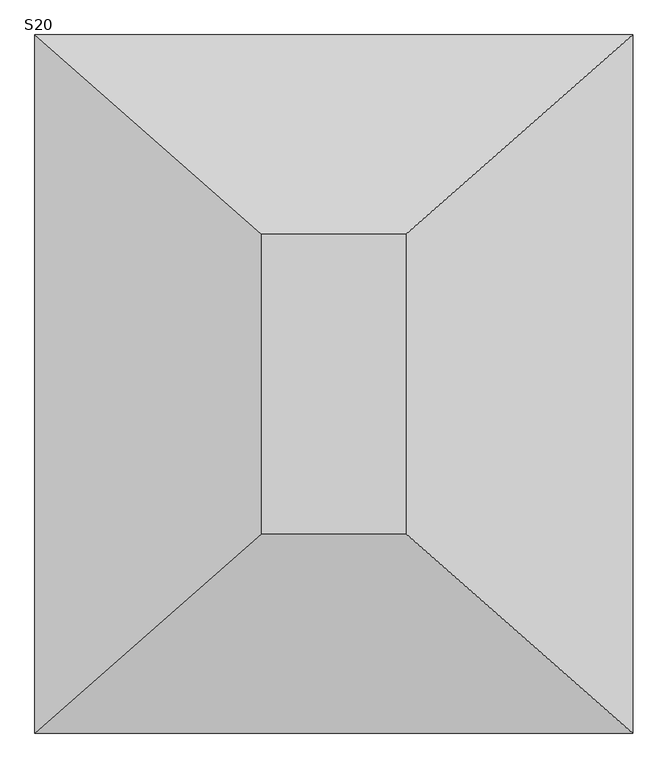
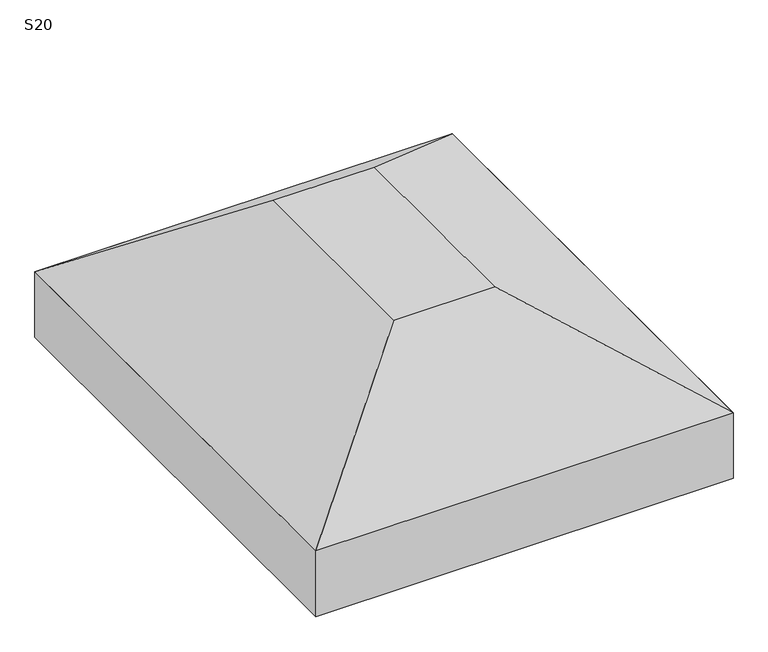
"""IFC4 building model written with IfcOpenShell, lengths in millimetres: fastener geometry, TQS - Sapata : S20."""

import ifcopenshell
import ifcopenshell.guid

model = None  # the IFC model being written
_history = None  # IfcOwnerHistory: only IFC2X3 demands one
_inside = {}  # id of a spatial element -> (the spatial element, [elements in it])
_under = {}  # id of a project, library or spatial element -> (it, [spatial elements below it])
_declared = {}  # id of a project -> (the project, [libraries it declares])
_typed = {}  # id of a type object -> (the type object, [elements of that type])
_made_of = {}  # id of a material, layer set ... -> (it, [elements and type objects made of it])


def new_model(schema):
    """Start an empty IFC model of exactly this schema.

    Asked for "IFC4X3", IfcOpenShell would pick the latest addendum, in which some entities
    have other attributes; the version numbers below select the first issue.
    IFC2X3 requires an IfcOwnerHistory on every rooted entity: one is made here for all.
    """
    global model, _history
    if schema == "IFC4X3":
        model = ifcopenshell.file(schema_version=(4, 3, 0, 0))
    else:
        model = ifcopenshell.file(schema=schema)
    _inside.clear()
    _under.clear()
    _declared.clear()
    _typed.clear()
    _made_of.clear()
    _history = None
    if model.schema == "IFC2X3":
        org = make("IfcOrganization", Name="unknown")
        user = make(
            "IfcPersonAndOrganization",
            ThePerson=make("IfcPerson", FamilyName="unknown"),
            TheOrganization=org,
        )
        app = make(
            "IfcApplication",
            ApplicationDeveloper=org,
            Version="unknown",
            ApplicationFullName="unknown",
            ApplicationIdentifier="unknown",
        )
        _history = make(
            "IfcOwnerHistory",
            OwningUser=user,
            OwningApplication=app,
            ChangeAction="ADDED",
            CreationDate=0,
        )
    return model


def make(cls, **values):
    """One entity of the class cls with the attributes given. An attribute that is None is left unset."""
    return model.create_entity(
        cls, **{name: value for name, value in values.items() if value is not None}
    )


def rooted(cls, **values):
    """An entity with a GlobalId (a new one), such as an element, a storey or a relation."""
    return make(cls, GlobalId=ifcopenshell.guid.new(), OwnerHistory=_history, **values)


def si_unit(unit_type, name, prefix=None):
    """IfcSIUnit, for example si_unit("LENGTHUNIT", "METRE", prefix="MILLI")."""
    return make("IfcSIUnit", UnitType=unit_type, Prefix=prefix, Name=name)


def assignment(units):
    """IfcUnitAssignment: the units of a project."""
    return None if units is None else make("IfcUnitAssignment", Units=units)


def point(xyz):
    """IfcCartesianPoint."""
    return None if xyz is None else make("IfcCartesianPoint", Coordinates=xyz)


def direction(xyz):
    """IfcDirection."""
    return None if xyz is None else make("IfcDirection", DirectionRatios=xyz)


def frame(location, z_axis=None, x_axis=None):
    """IfcAxis2Placement3D, a coordinate frame: its origin and axes. An axis left out is left unset."""
    return make(
        "IfcAxis2Placement3D",
        Location=point(location),
        Axis=direction(z_axis),
        RefDirection=direction(x_axis),
    )


def origin():
    """The frame at (0, 0, 0) with its axes left unset."""
    return frame((0.0, 0.0, 0.0))


def place(relative_to, where):
    """IfcLocalPlacement: puts the frame where relative to a parent placement (None: the world)."""
    return make(
        "IfcLocalPlacement", PlacementRelTo=relative_to, RelativePlacement=where
    )


def context(
    kind, dimensions, precision=None, world=None, true_north=None, identifier=None
):
    """IfcGeometricRepresentationContext, for example the 3D "Model" context."""
    return make(
        "IfcGeometricRepresentationContext",
        ContextIdentifier=identifier,
        ContextType=kind,
        CoordinateSpaceDimension=dimensions,
        Precision=precision,
        WorldCoordinateSystem=world,
        TrueNorth=true_north,
    )


def project(units=None, contexts=None):
    """IfcProject with its units and contexts."""
    return rooted(
        "IfcProject",
        Name="project",
        RepresentationContexts=contexts,
        UnitsInContext=assignment(units),
    )


def spatial(cls, under=None, at=None, **own):
    """A site, building, storey or space (cls), placed at a placement, below another one or the project."""
    s = rooted(cls, ObjectPlacement=at, **own)
    if under is not None:
        _under.setdefault(under.id(), (under, []))[1].append(s)
    return s


def polyline(points):
    """IfcPolyline through the points."""
    return make("IfcPolyline", Points=[point(p) for p in points])


def outline(outer, holes=None, kind="AREA"):
    """IfcArbitraryClosedProfileDef: a profile drawn as a closed curve; with holes, ...WithVoids."""
    if holes is None:
        return make("IfcArbitraryClosedProfileDef", ProfileType=kind, OuterCurve=outer)
    return make(
        "IfcArbitraryProfileDefWithVoids",
        ProfileType=kind,
        OuterCurve=outer,
        InnerCurves=holes,
    )


def extrude(swept, where, along, depth):
    """IfcExtrudedAreaSolid: the profile swept, set in the frame where, extruded along a direction by depth."""
    return make(
        "IfcExtrudedAreaSolid",
        SweptArea=swept,
        Position=where,
        ExtrudedDirection=direction(along),
        Depth=depth,
    )


def faces_of(points, faces, orient=None, outer=None):
    """IfcFace entities. A face is a list of loops; a loop is a list of indices into points, from 0.

    orient and outer hold one flag for each loop. By default every Orientation is true, the
    first loop of a face is its IfcFaceOuterBound and the others are IfcFaceBound.
    """
    made = []
    for i, loops in enumerate(faces):
        bounds = []
        for j, loop in enumerate(loops):
            is_outer = j == 0 if outer is None else outer[i][j]
            bounds.append(
                make(
                    "IfcFaceOuterBound" if is_outer else "IfcFaceBound",
                    Bound=make("IfcPolyLoop", Polygon=[points[k] for k in loop]),
                    Orientation=True if orient is None else orient[i][j],
                )
            )
        made.append(make("IfcFace", Bounds=bounds))
    return made


def faceted_brep(points, faces, orient=None, outer=None, voids=None):
    """IfcFacetedBrep: a solid bounded by flat faces; with voids (closed shells), ...WithVoids."""
    shared = [point(p) for p in points]
    hull = make("IfcClosedShell", CfsFaces=faces_of(shared, faces, orient, outer))
    if voids is None:
        return make("IfcFacetedBrep", Outer=hull)
    return make(
        "IfcFacetedBrepWithVoids",
        Outer=hull,
        Voids=[
            make(cls, CfsFaces=faces_of(shared, fs, o, b)) for cls, fs, o, b in voids
        ],
    )


def shape(context_of_items, identifier, shape_type, items):
    """IfcShapeRepresentation: the items that make up one representation, for example the "Body"."""
    return make(
        "IfcShapeRepresentation",
        ContextOfItems=context_of_items,
        RepresentationIdentifier=identifier,
        RepresentationType=shape_type,
        Items=items,
    )


def source(mapping_origin, context_of_items, identifier, shape_type, items):
    """IfcRepresentationMap: a shape defined once, which mapped items show again and again."""
    return make(
        "IfcRepresentationMap",
        MappingOrigin=mapping_origin,
        MappedRepresentation=shape(context_of_items, identifier, shape_type, items),
    )


def transform(
    local_origin,
    x_axis=None,
    y_axis=None,
    z_axis=None,
    scale=None,
    scale2=None,
    scale3=None,
    uniform=True,
):
    """IfcCartesianTransformationOperator3D, or its non-uniform kind. x_axis, y_axis, z_axis: its Axis1, 2, 3."""
    if uniform:
        return make(
            "IfcCartesianTransformationOperator3D",
            Axis1=direction(x_axis),
            Axis2=direction(y_axis),
            LocalOrigin=point(local_origin),
            Scale=scale,
            Axis3=direction(z_axis),
        )
    return make(
        "IfcCartesianTransformationOperator3DnonUniform",
        Axis1=direction(x_axis),
        Axis2=direction(y_axis),
        LocalOrigin=point(local_origin),
        Scale=scale,
        Axis3=direction(z_axis),
        Scale2=scale2,
        Scale3=scale3,
    )


def mapped(mapping_source, mapping_target):
    """IfcMappedItem: shows the shape of a source again, moved by a transform."""
    return make(
        "IfcMappedItem", MappingSource=mapping_source, MappingTarget=mapping_target
    )


def made_of(thing, what):
    """Note that an element or type object is made of a material, layer set ...; save() writes the relation."""
    if what is not None:
        _made_of.setdefault(what.id(), (what, []))[1].append(thing)
    return thing


def element(
    cls,
    number,
    at=None,
    inside=None,
    cuts=None,
    type_object=None,
    material=None,
    context=None,
    identifier="Body",
    shape_type=None,
    held_by="IfcProductDefinitionShape",
    body=None,
    shapes=None,
    **own,
):
    """One element of the class cls, such as IfcWall. Its Tag is "e" and its number.

    at: its placement. inside: the storey or other place that contains it. cuts: it is an
    opening in that element (IfcRelVoidsElement). A single representation is given by context,
    identifier, shape_type and body (its items); several are given by shapes. held_by: the class
    of the entity that holds the representations. save() writes the other relations.
    """
    e = rooted(cls, Tag="e%d" % number, ObjectPlacement=at, **own)
    if body is not None:
        shapes = [shape(context, identifier, shape_type, body)]
    if shapes is not None:
        e.Representation = make(held_by, Representations=shapes)
    if inside is not None:
        _inside.setdefault(inside.id(), (inside, []))[1].append(e)
    if cuts is not None:
        rooted(
            "IfcRelVoidsElement", RelatingBuildingElement=cuts, RelatedOpeningElement=e
        )
    if type_object is not None:
        _typed.setdefault(type_object.id(), (type_object, []))[1].append(e)
    return made_of(e, material)


def aggregate(whole, parts):
    """IfcRelAggregates: a whole, such as a stair, and the parts it consists of."""
    return rooted("IfcRelAggregates", RelatingObject=whole, RelatedObjects=parts)


def save(model, path):
    """Write the relations noted so far, then the file.

    IfcRelAggregates (storeys below a building ...), IfcRelContainedInSpatialStructure (elements
    in a storey), IfcRelDefinesByType, IfcRelAssociatesMaterial and IfcRelDeclares: one each for
    every whole, place, type object, material and project.
    """
    for whole, parts in _under.values():
        aggregate(whole, parts)
    for where, things in _inside.values():
        rooted(
            "IfcRelContainedInSpatialStructure",
            RelatedElements=things,
            RelatingStructure=where,
        )
    for kind, things in _typed.values():
        rooted("IfcRelDefinesByType", RelatedObjects=things, RelatingType=kind)
    for what, things in _made_of.values():
        rooted("IfcRelAssociatesMaterial", RelatedObjects=things, RelatingMaterial=what)
    for by, libraries in _declared.values():
        rooted("IfcRelDeclares", RelatingContext=by, RelatedDefinitions=libraries)
    model.write(path)


def s20_c409a0c5(model_context):
    return source(origin(), model_context, "Body", "SolidModel", [
        faceted_brep([(-55.0, 100.0, 0.0), (-345.0, 100.0, 0.0), (-345.0, -500.0, 0.0), (-55.0, -500.0, 0.0), (400.0, 500.0, -300.0), (400.0, -900.0, -300.0), (-800.0, -900.0, -300.0), (-800.0, 500.0, -300.0)], [[[0, 1, 2, 3]], [[4, 5, 6, 7]], [[4, 7, 1, 0]], [[7, 6, 2, 1]], [[6, 5, 3, 2]], [[5, 4, 0, 3]]]),
        extrude(outline(polyline([(400.0, 500.0), (400.0, -900.0), (-800.0, -900.0), (-800.0, 500.0), (400.0, 500.0)])), frame((0.0, 0.0, -500.0), z_axis=(0.0, 0.0, 1.0), x_axis=(1.0, 0.0, 0.0)), (0.0, 0.0, 1.0), 200.0),
    ])


if __name__ == "__main__":
    model = new_model("IFC4")
    model_context = context("Model", 3, world=origin())
    ifc_project = project(units=[si_unit("LENGTHUNIT", "METRE", prefix="MILLI")], contexts=[model_context])
    site = spatial("IfcSite", under=ifc_project)
    building = spatial("IfcBuilding", under=site)
    placement = place(None, origin())
    s20_shape = s20_c409a0c5(model_context)
    element("IfcFastener", 1, ObjectType="TQS - Sapata : S20", at=placement, inside=building, context=model_context, shape_type="MappedRepresentation", body=[
        mapped(s20_shape, transform((0.0, 0.0, 0.0), x_axis=(1.0, 0.0, 0.0), y_axis=(0.0, 1.0, 0.0), z_axis=(0.0, 0.0, 1.0))),
    ])
    save(model, "model.ifc")

# Revit data of these elements
# Type "TQS - Sapata : S20"
#   TY = 0.60 m
#   TX = 0.29 m
#   HS = 0.50 m
#   H0 = 0.20 m
#   EXCYABS = 0.70 m
#   EXCY = 0.00 m
#   EXCXABS = 0.60 m
#   EXCX = 0.00 m
#   DIMY = 1.40 m
#   DIMX = 1.20 m
#   Material estrutural = Concreto - Concreto concretado no local
#   Width = 0
#   Length = 0
# Element 1 (IfcFastener, "TQS - Sapata : S20")
#   Materials on its faces: "Concreto - Concreto concretado no local"
# Materials
#   "Concreto - Concreto concretado no local": class "Concreto", colour RGB 192 192 192, transparency 0
